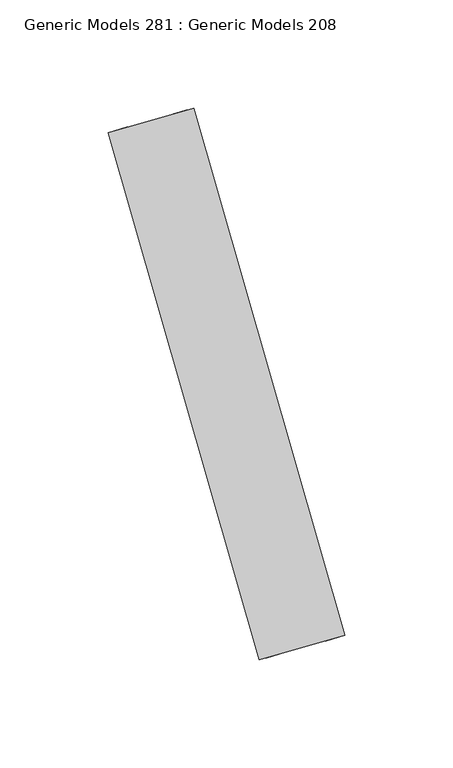
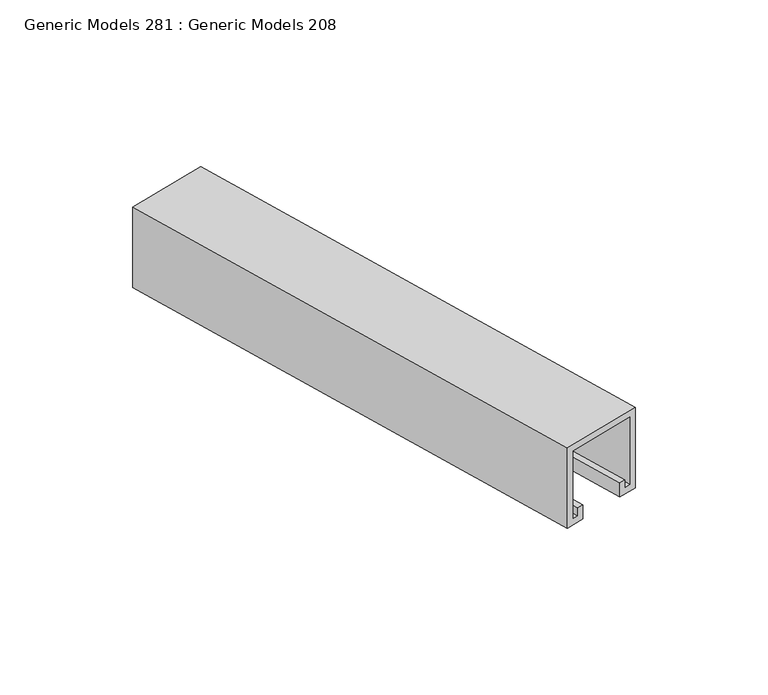
"""IFC4 building model written with IfcOpenShell, lengths in millimetres: proxy geometry, Generic Models 281 : Generic Models 208."""

from ifc_helpers import new_model, si_unit, frame, origin, place, context, project, spatial, polyline, outline, extrude, source, transform, mapped, element, save


def generic_models_281_generic_models_208_16d38fc9(model_context):
    return source(origin(), model_context, "Body", "SweptSolid", [
        extrude(outline(polyline([(-3.175, 0.0), (-3.175, 34.925), (-38.1, 34.925), (-38.1, 31.7500001), (-34.13125, 31.7500001), (-34.13125, 28.575), (-41.275, 28.575), (-41.275, 38.1), (0.0, 38.1), (0.0, -3.1749999), (-41.275, -3.1749999), (-41.275, 6.3500001), (-34.13125, 6.3500001), (-34.13125, 3.175), (-38.1, 3.175), (-38.1, 0.0), (-3.175, 0.0)])), frame((-1631.6619367, -22413.5661163, 1035.05), z_axis=(-0.2755378426876231, 0.9612902252946561, 0.0), x_axis=(0.0, 0.0, 1.0)), (0.0, 0.0, 1.0), 254.0),
    ])


if __name__ == "__main__":
    model = new_model("IFC4")
    model_context = context("Model", 3, world=origin())
    ifc_project = project(units=[si_unit("LENGTHUNIT", "METRE", prefix="MILLI")], contexts=[model_context])
    site = spatial("IfcSite", under=ifc_project)
    building = spatial("IfcBuilding", under=site)
    placement = place(None, origin())
    generic_models_281_generic_models_208_shape = generic_models_281_generic_models_208_16d38fc9(model_context)
    element("IfcBuildingElementProxy", 1, Name="Generic Models 281 : Generic Models 208", ObjectType="Generic Models 281 : Generic Models 208", at=placement, inside=building, context=model_context, shape_type="MappedRepresentation", body=[
        mapped(generic_models_281_generic_models_208_shape, transform((0.0, 0.0, 0.0), x_axis=(1.0, 0.0, 0.0), y_axis=(0.0, 1.0, 0.0), z_axis=(0.0, 0.0, 1.0))),
    ])
    save(model, "model.ifc")

# Revit data of these elements
# Element 1 (IfcBuildingElementProxy, "Generic Models 281 : Generic Models 208")
#   Materials on its faces: "UNISTRUT P1000, 1 5/8\" X 1 5/8\", CHANNEL OR ALUM. CHANNEL"
# Materials
#   "UNISTRUT P1000, 1 5/8\" X 1 5/8\", CHANNEL OR ALUM. CHANNEL": class "Metal", colour RGB 244 244 244, transparency 0, Description = "Aluminum 6061", Cost = 0
